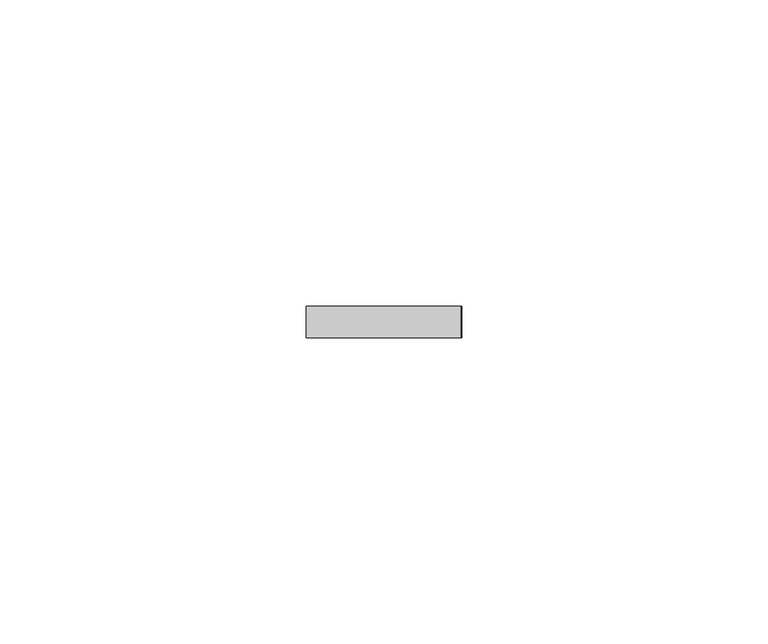
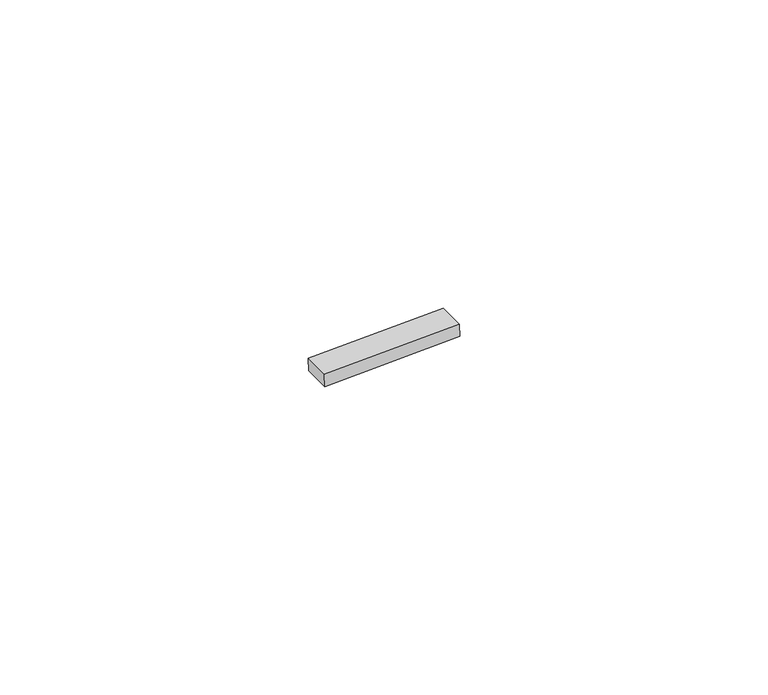
"""IFC4 building model written with IfcOpenShell, lengths in millimetres: proxy geometry, Inner panel:Inner panel:1:Inner panel:1 : Inner panel:Inner panel:300324:2:Inner panel:1:Inner panel:1 : Inner panel:Inner panel:300324:2 : Inner panel:Inner panel:1:Inner panel:1 : Inner panel:Inner panel:300324:300043:145 : Inner panel:Inner panel:1:Inner panel:1 : Inner panel:Inner panel:300324:2:Inner panel:1:Inner panel:1 : Inner panel:Inner panel:300324:2 : Inner panel:Inner panel:1:Inner panel:1 : Inner panel:Inner panel:300324:300043:308120."""

from ifc_helpers import new_model, si_unit, frame, origin, place, context, project, spatial, polyline, outline, extrude, source, transform, mapped, element, save


def generic_models_cd309641(model_context):
    return source(origin(), model_context, "Body", "SweptSolid", [
        extrude(outline(polyline([(0.0, -25.3999999), (0.0, 0.0), (5.2138089, 0.0), (5.2138089, -25.3999999), (0.0, -25.3999999)])), frame((558903.2033258, -578534.9848948, 3888.9625848), z_axis=(-0.041630544712223896, 0.0, 0.9991330730923502), x_axis=(0.0, -1.0, 0.0)), (0.0, 0.0, 1.0), 2.4763745),
    ])


if __name__ == "__main__":
    model = new_model("IFC4")
    model_context = context("Model", 3, world=origin())
    ifc_project = project(units=[si_unit("LENGTHUNIT", "METRE", prefix="MILLI")], contexts=[model_context])
    site = spatial("IfcSite", under=ifc_project)
    building = spatial("IfcBuilding", under=site)
    placement = place(None, origin())
    generic_models_shape = generic_models_cd309641(model_context)
    element("IfcBuildingElementProxy", 1, Name="Inner panel:Inner panel:1:Inner panel:1 : Inner panel:Inner panel:300324:2:Inner panel:1:Inner panel:1 : Inner panel:Inner panel:300324:2 : Inner panel:Inner panel:1:Inner panel:1 : Inner panel:Inner panel:300324:300043:145 : Inner panel:Inner panel:1:Inner panel:1 : Inner panel:Inner panel:300324:2:Inner panel:1:Inner panel:1 : Inner panel:Inner panel:300324:2 : Inner panel:Inner panel:1:Inner panel:1 : Inner panel:Inner panel:300324:300043:308120", ObjectType="Inner panel:Inner panel:1:Inner panel:1 : Inner panel:Inner panel:300324:2:Inner panel:1:Inner panel:1 : Inner panel:Inner panel:300324:2 : Inner panel:Inner panel:1:Inner panel:1 : Inner panel:Inner panel:300324:300043:145 : Inner panel:Inner panel:1:Inner panel:1 : Inner panel:Inner panel:300324:2:Inner panel:1:Inner panel:1 : Inner panel:Inner panel:300324:2 : Inner panel:Inner panel:1:Inner panel:1 : Inner panel:Inner panel:300324:300043:308120", at=placement, inside=building, context=model_context, shape_type="MappedRepresentation", body=[
        mapped(generic_models_shape, transform((0.0, 0.0, 0.0), x_axis=(1.0, 0.0, 0.0), y_axis=(0.0, 1.0, 0.0), z_axis=(0.0, 0.0, 1.0))),
    ])
    save(model, "model.ifc")

# Revit data of these elements
# Type "Inner panel:Inner panel:1:Inner panel:1 : Inner panel:Inner panel:300324:2:Inner panel:1:Inner panel:1 : Inner panel:Inner panel:300324:2 : Inner panel:Inner panel:1:Inner panel:1 : Inner panel:Inner panel:300324:300043:145 : Inner panel:Inner panel:1:Inner panel:1 : Inner panel:Inner panel:300324:2:Inner panel:1:Inner panel:1 : Inner panel:Inner panel:300324:2 : Inner panel:Inner panel:1:Inner panel:1 : Inner panel:Inner panel:300324:300043:308120"
#   NameOverride = "Inner panel:Inner panel:1:Inner panel:1 : Inner panel:Inner panel:300324:2:Inner panel:1:Inner panel:1 : Inner panel:Inner panel:300324:2 : Inner panel:Inner panel:1:Inner panel:1 : Inner panel:Inner panel:300324:300043:308120"
#   ObjectTypeOverride = "Inner panel:1:Inner panel:1 : Inner panel:Inner panel:300324:2 : Inner panel:Inner panel:1:Inner panel:1 : Inner panel:Inner panel:300324:300043"
#   Reference = "Inner panel"
#   Tag = "308120"
# Element 1 (IfcBuildingElementProxy, "Inner panel:Inner panel:1:Inner panel:1 : Inner panel:Inner panel:300324:2:Inner panel:1:Inner panel:1 : Inner panel:Inner panel:300324:2 : Inner panel:Inner panel:1:Inner panel:1 : Inner panel:Inner panel:300324:300043:145 : Inner panel:Inner panel:1:Inner panel:1 : Inner panel:Inner panel:300324:2:Inner panel:1:Inner panel:1 : Inner panel:Inner panel:300324:2 : Inner panel:Inner panel:1:Inner panel:1 : Inner panel:Inner panel:300324:300043:308120")
#   Materials on its faces: "AT CLIP - 1\" WIDE NON ABSORBENT, WEATHER-RESISTANT NEOPRENE/EPDM/SBR FOAM"
# Materials
#   "AT CLIP - 1\" WIDE NON ABSORBENT, WEATHER-RESISTANT NEOPRENE/EPDM/SBR FOAM": class "Generic", colour RGB 85 85 85, transparency 0, Cost = 0
